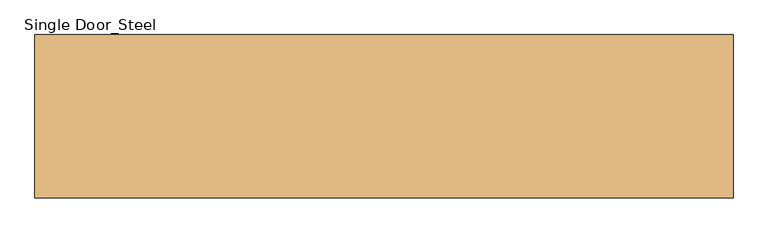
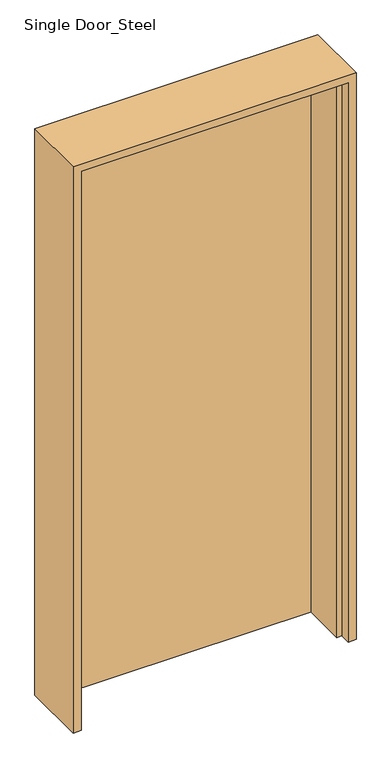
"""IFC4 building model written with IfcOpenShell, lengths in millimetres: door geometry, Single Door_Steel : H_DR_AR B12_Door_Single_W1100xH2280_FR 1.0H_FSD-2."""

import ifcopenshell
import ifcopenshell.guid

model = None  # the IFC model being written
_history = None  # IfcOwnerHistory: only IFC2X3 demands one
_inside = {}  # id of a spatial element -> (the spatial element, [elements in it])
_under = {}  # id of a project, library or spatial element -> (it, [spatial elements below it])
_declared = {}  # id of a project -> (the project, [libraries it declares])
_typed = {}  # id of a type object -> (the type object, [elements of that type])
_made_of = {}  # id of a material, layer set ... -> (it, [elements and type objects made of it])


def new_model(schema):
    """Start an empty IFC model of exactly this schema.

    Asked for "IFC4X3", IfcOpenShell would pick the latest addendum, in which some entities
    have other attributes; the version numbers below select the first issue.
    IFC2X3 requires an IfcOwnerHistory on every rooted entity: one is made here for all.
    """
    global model, _history
    if schema == "IFC4X3":
        model = ifcopenshell.file(schema_version=(4, 3, 0, 0))
    else:
        model = ifcopenshell.file(schema=schema)
    _inside.clear()
    _under.clear()
    _declared.clear()
    _typed.clear()
    _made_of.clear()
    _history = None
    if model.schema == "IFC2X3":
        org = make("IfcOrganization", Name="unknown")
        user = make(
            "IfcPersonAndOrganization",
            ThePerson=make("IfcPerson", FamilyName="unknown"),
            TheOrganization=org,
        )
        app = make(
            "IfcApplication",
            ApplicationDeveloper=org,
            Version="unknown",
            ApplicationFullName="unknown",
            ApplicationIdentifier="unknown",
        )
        _history = make(
            "IfcOwnerHistory",
            OwningUser=user,
            OwningApplication=app,
            ChangeAction="ADDED",
            CreationDate=0,
        )
    return model


def make(cls, **values):
    """One entity of the class cls with the attributes given. An attribute that is None is left unset."""
    return model.create_entity(
        cls, **{name: value for name, value in values.items() if value is not None}
    )


def rooted(cls, **values):
    """An entity with a GlobalId (a new one), such as an element, a storey or a relation."""
    return make(cls, GlobalId=ifcopenshell.guid.new(), OwnerHistory=_history, **values)


def si_unit(unit_type, name, prefix=None):
    """IfcSIUnit, for example si_unit("LENGTHUNIT", "METRE", prefix="MILLI")."""
    return make("IfcSIUnit", UnitType=unit_type, Prefix=prefix, Name=name)


def assignment(units):
    """IfcUnitAssignment: the units of a project."""
    return None if units is None else make("IfcUnitAssignment", Units=units)


def point(xyz):
    """IfcCartesianPoint."""
    return None if xyz is None else make("IfcCartesianPoint", Coordinates=xyz)


def direction(xyz):
    """IfcDirection."""
    return None if xyz is None else make("IfcDirection", DirectionRatios=xyz)


def frame(location, z_axis=None, x_axis=None):
    """IfcAxis2Placement3D, a coordinate frame: its origin and axes. An axis left out is left unset."""
    return make(
        "IfcAxis2Placement3D",
        Location=point(location),
        Axis=direction(z_axis),
        RefDirection=direction(x_axis),
    )


def origin():
    """The frame at (0, 0, 0) with its axes left unset."""
    return frame((0.0, 0.0, 0.0))


def origin_with_axes():
    """The frame at (0, 0, 0) with the z axis (0, 0, 1) and the x axis (1, 0, 0) written out."""
    return frame((0.0, 0.0, 0.0), z_axis=(0.0, 0.0, 1.0), x_axis=(1.0, 0.0, 0.0))


def place(relative_to, where):
    """IfcLocalPlacement: puts the frame where relative to a parent placement (None: the world)."""
    return make(
        "IfcLocalPlacement", PlacementRelTo=relative_to, RelativePlacement=where
    )


def context(
    kind, dimensions, precision=None, world=None, true_north=None, identifier=None
):
    """IfcGeometricRepresentationContext, for example the 3D "Model" context."""
    return make(
        "IfcGeometricRepresentationContext",
        ContextIdentifier=identifier,
        ContextType=kind,
        CoordinateSpaceDimension=dimensions,
        Precision=precision,
        WorldCoordinateSystem=world,
        TrueNorth=true_north,
    )


def project(units=None, contexts=None):
    """IfcProject with its units and contexts."""
    return rooted(
        "IfcProject",
        Name="project",
        RepresentationContexts=contexts,
        UnitsInContext=assignment(units),
    )


def spatial(cls, under=None, at=None, **own):
    """A site, building, storey or space (cls), placed at a placement, below another one or the project."""
    s = rooted(cls, ObjectPlacement=at, **own)
    if under is not None:
        _under.setdefault(under.id(), (under, []))[1].append(s)
    return s


def polyline(points):
    """IfcPolyline through the points."""
    return make("IfcPolyline", Points=[point(p) for p in points])


def outline(outer, holes=None, kind="AREA"):
    """IfcArbitraryClosedProfileDef: a profile drawn as a closed curve; with holes, ...WithVoids."""
    if holes is None:
        return make("IfcArbitraryClosedProfileDef", ProfileType=kind, OuterCurve=outer)
    return make(
        "IfcArbitraryProfileDefWithVoids",
        ProfileType=kind,
        OuterCurve=outer,
        InnerCurves=holes,
    )


def extrude(swept, where, along, depth):
    """IfcExtrudedAreaSolid: the profile swept, set in the frame where, extruded along a direction by depth."""
    return make(
        "IfcExtrudedAreaSolid",
        SweptArea=swept,
        Position=where,
        ExtrudedDirection=direction(along),
        Depth=depth,
    )


def faces_of(points, faces, orient=None, outer=None):
    """IfcFace entities. A face is a list of loops; a loop is a list of indices into points, from 0.

    orient and outer hold one flag for each loop. By default every Orientation is true, the
    first loop of a face is its IfcFaceOuterBound and the others are IfcFaceBound.
    """
    made = []
    for i, loops in enumerate(faces):
        bounds = []
        for j, loop in enumerate(loops):
            is_outer = j == 0 if outer is None else outer[i][j]
            bounds.append(
                make(
                    "IfcFaceOuterBound" if is_outer else "IfcFaceBound",
                    Bound=make("IfcPolyLoop", Polygon=[points[k] for k in loop]),
                    Orientation=True if orient is None else orient[i][j],
                )
            )
        made.append(make("IfcFace", Bounds=bounds))
    return made


def faceted_brep(points, faces, orient=None, outer=None, voids=None):
    """IfcFacetedBrep: a solid bounded by flat faces; with voids (closed shells), ...WithVoids."""
    shared = [point(p) for p in points]
    hull = make("IfcClosedShell", CfsFaces=faces_of(shared, faces, orient, outer))
    if voids is None:
        return make("IfcFacetedBrep", Outer=hull)
    return make(
        "IfcFacetedBrepWithVoids",
        Outer=hull,
        Voids=[
            make(cls, CfsFaces=faces_of(shared, fs, o, b)) for cls, fs, o, b in voids
        ],
    )


def shape(context_of_items, identifier, shape_type, items):
    """IfcShapeRepresentation: the items that make up one representation, for example the "Body"."""
    return make(
        "IfcShapeRepresentation",
        ContextOfItems=context_of_items,
        RepresentationIdentifier=identifier,
        RepresentationType=shape_type,
        Items=items,
    )


def source(mapping_origin, context_of_items, identifier, shape_type, items):
    """IfcRepresentationMap: a shape defined once, which mapped items show again and again."""
    return make(
        "IfcRepresentationMap",
        MappingOrigin=mapping_origin,
        MappedRepresentation=shape(context_of_items, identifier, shape_type, items),
    )


def transform(
    local_origin,
    x_axis=None,
    y_axis=None,
    z_axis=None,
    scale=None,
    scale2=None,
    scale3=None,
    uniform=True,
):
    """IfcCartesianTransformationOperator3D, or its non-uniform kind. x_axis, y_axis, z_axis: its Axis1, 2, 3."""
    if uniform:
        return make(
            "IfcCartesianTransformationOperator3D",
            Axis1=direction(x_axis),
            Axis2=direction(y_axis),
            LocalOrigin=point(local_origin),
            Scale=scale,
            Axis3=direction(z_axis),
        )
    return make(
        "IfcCartesianTransformationOperator3DnonUniform",
        Axis1=direction(x_axis),
        Axis2=direction(y_axis),
        LocalOrigin=point(local_origin),
        Scale=scale,
        Axis3=direction(z_axis),
        Scale2=scale2,
        Scale3=scale3,
    )


def mapped(mapping_source, mapping_target):
    """IfcMappedItem: shows the shape of a source again, moved by a transform."""
    return make(
        "IfcMappedItem", MappingSource=mapping_source, MappingTarget=mapping_target
    )


def made_of(thing, what):
    """Note that an element or type object is made of a material, layer set ...; save() writes the relation."""
    if what is not None:
        _made_of.setdefault(what.id(), (what, []))[1].append(thing)
    return thing


def element(
    cls,
    number,
    at=None,
    inside=None,
    cuts=None,
    type_object=None,
    material=None,
    context=None,
    identifier="Body",
    shape_type=None,
    held_by="IfcProductDefinitionShape",
    body=None,
    shapes=None,
    **own,
):
    """One element of the class cls, such as IfcWall. Its Tag is "e" and its number.

    at: its placement. inside: the storey or other place that contains it. cuts: it is an
    opening in that element (IfcRelVoidsElement). A single representation is given by context,
    identifier, shape_type and body (its items); several are given by shapes. held_by: the class
    of the entity that holds the representations. save() writes the other relations.
    """
    e = rooted(cls, Tag="e%d" % number, ObjectPlacement=at, **own)
    if body is not None:
        shapes = [shape(context, identifier, shape_type, body)]
    if shapes is not None:
        e.Representation = make(held_by, Representations=shapes)
    if inside is not None:
        _inside.setdefault(inside.id(), (inside, []))[1].append(e)
    if cuts is not None:
        rooted(
            "IfcRelVoidsElement", RelatingBuildingElement=cuts, RelatedOpeningElement=e
        )
    if type_object is not None:
        _typed.setdefault(type_object.id(), (type_object, []))[1].append(e)
    return made_of(e, material)


def aggregate(whole, parts):
    """IfcRelAggregates: a whole, such as a stair, and the parts it consists of."""
    return rooted("IfcRelAggregates", RelatingObject=whole, RelatedObjects=parts)


def save(model, path):
    """Write the relations noted so far, then the file.

    IfcRelAggregates (storeys below a building ...), IfcRelContainedInSpatialStructure (elements
    in a storey), IfcRelDefinesByType, IfcRelAssociatesMaterial and IfcRelDeclares: one each for
    every whole, place, type object, material and project.
    """
    for whole, parts in _under.values():
        aggregate(whole, parts)
    for where, things in _inside.values():
        rooted(
            "IfcRelContainedInSpatialStructure",
            RelatedElements=things,
            RelatingStructure=where,
        )
    for kind, things in _typed.values():
        rooted("IfcRelDefinesByType", RelatedObjects=things, RelatingType=kind)
    for what, things in _made_of.values():
        rooted("IfcRelAssociatesMaterial", RelatedObjects=things, RelatingMaterial=what)
    for by, libraries in _declared.values():
        rooted("IfcRelDeclares", RelatingContext=by, RelatedDefinitions=libraries)
    model.write(path)


def single_door_steel_78a4d33a(model_context):
    return source(origin(), model_context, "Body", "SolidModel", [
        extrude(outline(polyline([(505.0, 125.0), (505.0, 85.0), (-505.0, 85.0), (-505.0, 125.0), (505.0, 125.0)])), origin_with_axes(), (0.0, 0.0, 1.0), 2235.0),
        faceted_brep([(505.0, 125.0, 0.0), (535.0, 125.0, 0.0), (535.0, -125.0, 0.0), (505.0, -125.0, 0.0), (505.0, -85.0, 0.0), (485.0, -85.0, 0.0), (485.0, 85.0, 0.0), (505.0, 85.0, 0.0), (505.0, 125.0, 2235.0), (-505.0, 125.0, 2235.0), (-505.0, 125.0, 0.0), (-535.0, 125.0, 0.0), (-535.0, 125.0, 2265.0), (535.0, 125.0, 2265.0), (535.0, -125.0, 2265.0), (-535.0, -125.0, 2265.0), (-535.0, -125.0, 0.0), (-505.0, -125.0, 0.0), (-505.0, -125.0, 2235.0), (505.0, -125.0, 2235.0), (505.0, -85.0, 2235.0), (-505.0, -85.0, 2235.0), (-505.0, -85.0, 0.0), (-485.0, -85.0, 0.0), (-485.0, -85.0, 2215.0), (485.0, -85.0, 2215.0), (485.0, 85.0, 2215.0), (-485.0, 85.0, 2215.0), (-485.0, 85.0, 0.0), (-505.0, 85.0, 0.0), (-505.0, 85.0, 2235.0), (505.0, 85.0, 2235.0)], [[[0, 1, 2, 3, 4, 5, 6, 7]], [[1, 0, 8, 9, 10, 11, 12, 13]], [[2, 1, 13, 14]], [[3, 2, 14, 15, 16, 17, 18, 19]], [[4, 3, 19, 20]], [[5, 4, 20, 21, 22, 23, 24, 25]], [[6, 5, 25, 26]], [[7, 6, 26, 27, 28, 29, 30, 31]], [[0, 7, 31, 8]], [[9, 30, 29, 10]], [[10, 29, 28, 23, 22, 17, 16, 11]], [[15, 12, 11, 16]], [[21, 18, 17, 22]], [[27, 24, 23, 28]], [[14, 13, 12, 15]], [[20, 19, 18, 21]], [[26, 25, 24, 27]], [[8, 31, 30, 9]]]),
    ])


if __name__ == "__main__":
    model = new_model("IFC4")
    model_context = context("Model", 3, world=origin())
    ifc_project = project(units=[si_unit("LENGTHUNIT", "METRE", prefix="MILLI")], contexts=[model_context])
    site = spatial("IfcSite", under=ifc_project)
    building = spatial("IfcBuilding", under=site)
    placement = place(None, origin())
    single_door_steel_shape = single_door_steel_78a4d33a(model_context)
    element("IfcDoor", 1, ObjectType="Single Door_Steel : H_DR_AR B12_Door_Single_W1100xH2280_FR 1.0H_FSD-2", at=placement, inside=building, context=model_context, shape_type="MappedRepresentation", body=[
        mapped(single_door_steel_shape, transform((0.0, 0.0, 0.0), x_axis=(1.0, 0.0, 0.0), y_axis=(0.0, 1.0, 0.0), z_axis=(0.0, 0.0, 1.0))),
    ])
    save(model, "model.ifc")

# Revit data of these elements
# Type "Single Door_Steel : H_DR_AR B12_Door_Single_W1100xH2280_FR 1.0H_FSD-2"
#   Type Mark = "442"
#   Analytic Construction = "<None>"
#   프레임 투영 외부. = 25 mm
#   프레임 투영 내부. = 25 mm
#   프레임 폭 = 75 mm
#   Height = 2280 mm
#   Width = 1100 mm
#   Define Thermal Properties by = 1
#   문 패널 = none
#   문 프레임 = none
#   Function = (empty or 0)
#   Wall Closure = (empty or 0)
